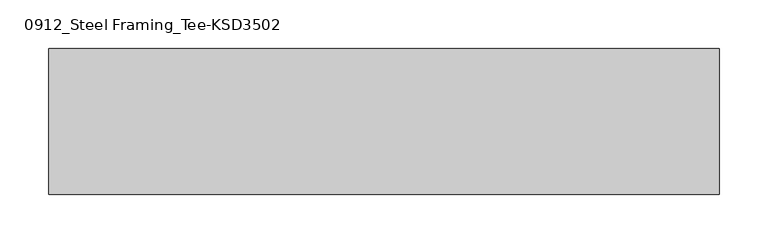
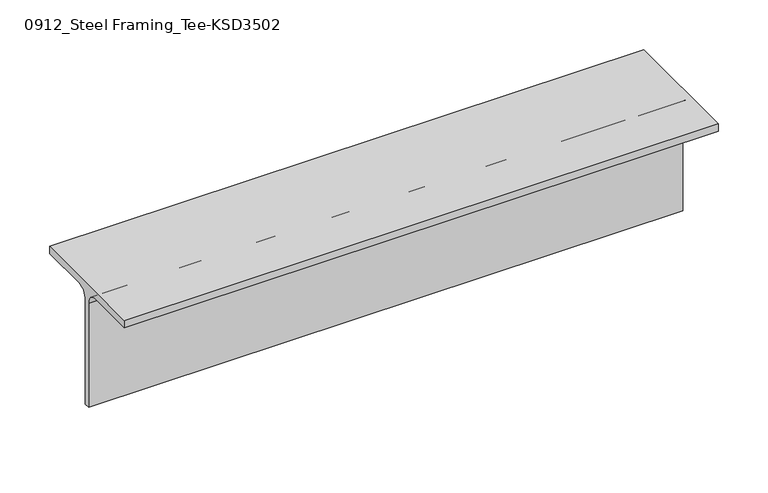
"""IFC4 building model written with IfcOpenShell, lengths in millimetres: member geometry, 0912_Steel Framing_Tee-KSD3502 : H_SB_ASB_CT-150x150x6.5x9."""

import ifcopenshell
import ifcopenshell.guid

model = None  # the IFC model being written
_history = None  # IfcOwnerHistory: only IFC2X3 demands one
_inside = {}  # id of a spatial element -> (the spatial element, [elements in it])
_under = {}  # id of a project, library or spatial element -> (it, [spatial elements below it])
_declared = {}  # id of a project -> (the project, [libraries it declares])
_typed = {}  # id of a type object -> (the type object, [elements of that type])
_made_of = {}  # id of a material, layer set ... -> (it, [elements and type objects made of it])


def new_model(schema):
    """Start an empty IFC model of exactly this schema.

    Asked for "IFC4X3", IfcOpenShell would pick the latest addendum, in which some entities
    have other attributes; the version numbers below select the first issue.
    IFC2X3 requires an IfcOwnerHistory on every rooted entity: one is made here for all.
    """
    global model, _history
    if schema == "IFC4X3":
        model = ifcopenshell.file(schema_version=(4, 3, 0, 0))
    else:
        model = ifcopenshell.file(schema=schema)
    _inside.clear()
    _under.clear()
    _declared.clear()
    _typed.clear()
    _made_of.clear()
    _history = None
    if model.schema == "IFC2X3":
        org = make("IfcOrganization", Name="unknown")
        user = make(
            "IfcPersonAndOrganization",
            ThePerson=make("IfcPerson", FamilyName="unknown"),
            TheOrganization=org,
        )
        app = make(
            "IfcApplication",
            ApplicationDeveloper=org,
            Version="unknown",
            ApplicationFullName="unknown",
            ApplicationIdentifier="unknown",
        )
        _history = make(
            "IfcOwnerHistory",
            OwningUser=user,
            OwningApplication=app,
            ChangeAction="ADDED",
            CreationDate=0,
        )
    return model


def make(cls, **values):
    """One entity of the class cls with the attributes given. An attribute that is None is left unset."""
    return model.create_entity(
        cls, **{name: value for name, value in values.items() if value is not None}
    )


def rooted(cls, **values):
    """An entity with a GlobalId (a new one), such as an element, a storey or a relation."""
    return make(cls, GlobalId=ifcopenshell.guid.new(), OwnerHistory=_history, **values)


def si_unit(unit_type, name, prefix=None):
    """IfcSIUnit, for example si_unit("LENGTHUNIT", "METRE", prefix="MILLI")."""
    return make("IfcSIUnit", UnitType=unit_type, Prefix=prefix, Name=name)


def assignment(units):
    """IfcUnitAssignment: the units of a project."""
    return None if units is None else make("IfcUnitAssignment", Units=units)


def point(xyz):
    """IfcCartesianPoint."""
    return None if xyz is None else make("IfcCartesianPoint", Coordinates=xyz)


def direction(xyz):
    """IfcDirection."""
    return None if xyz is None else make("IfcDirection", DirectionRatios=xyz)


def frame(location, z_axis=None, x_axis=None):
    """IfcAxis2Placement3D, a coordinate frame: its origin and axes. An axis left out is left unset."""
    return make(
        "IfcAxis2Placement3D",
        Location=point(location),
        Axis=direction(z_axis),
        RefDirection=direction(x_axis),
    )


def frame_2d(location, x_axis=None):
    """IfcAxis2Placement2D, a coordinate frame in the plane: its origin and x axis."""
    return make(
        "IfcAxis2Placement2D", Location=point(location), RefDirection=direction(x_axis)
    )


def origin():
    """The frame at (0, 0, 0) with its axes left unset."""
    return frame((0.0, 0.0, 0.0))


def place(relative_to, where):
    """IfcLocalPlacement: puts the frame where relative to a parent placement (None: the world)."""
    return make(
        "IfcLocalPlacement", PlacementRelTo=relative_to, RelativePlacement=where
    )


def context(
    kind, dimensions, precision=None, world=None, true_north=None, identifier=None
):
    """IfcGeometricRepresentationContext, for example the 3D "Model" context."""
    return make(
        "IfcGeometricRepresentationContext",
        ContextIdentifier=identifier,
        ContextType=kind,
        CoordinateSpaceDimension=dimensions,
        Precision=precision,
        WorldCoordinateSystem=world,
        TrueNorth=true_north,
    )


def project(units=None, contexts=None):
    """IfcProject with its units and contexts."""
    return rooted(
        "IfcProject",
        Name="project",
        RepresentationContexts=contexts,
        UnitsInContext=assignment(units),
    )


def spatial(cls, under=None, at=None, **own):
    """A site, building, storey or space (cls), placed at a placement, below another one or the project."""
    s = rooted(cls, ObjectPlacement=at, **own)
    if under is not None:
        _under.setdefault(under.id(), (under, []))[1].append(s)
    return s


def polyline(points):
    """IfcPolyline through the points."""
    return make("IfcPolyline", Points=[point(p) for p in points])


def circle_curve(where, radius):
    """IfcCircle in the frame where."""
    return make("IfcCircle", Position=where, Radius=radius)


def trimmed(basis, trim1, trim2, sense, master):
    """IfcTrimmedCurve: the piece of a basis curve between two trims."""
    return make(
        "IfcTrimmedCurve",
        BasisCurve=basis,
        Trim1=trim1,
        Trim2=trim2,
        SenseAgreement=sense,
        MasterRepresentation=master,
    )


def segment(curve, same_sense, transition):
    """IfcCompositeCurveSegment."""
    return make(
        "IfcCompositeCurveSegment",
        Transition=transition,
        SameSense=same_sense,
        ParentCurve=curve,
    )


def composite_curve(segments, self_intersect=None):
    """IfcCompositeCurve: segments joined end to end."""
    return make("IfcCompositeCurve", Segments=segments, SelfIntersect=self_intersect)


def outline(outer, holes=None, kind="AREA"):
    """IfcArbitraryClosedProfileDef: a profile drawn as a closed curve; with holes, ...WithVoids."""
    if holes is None:
        return make("IfcArbitraryClosedProfileDef", ProfileType=kind, OuterCurve=outer)
    return make(
        "IfcArbitraryProfileDefWithVoids",
        ProfileType=kind,
        OuterCurve=outer,
        InnerCurves=holes,
    )


def extrude(swept, where, along, depth):
    """IfcExtrudedAreaSolid: the profile swept, set in the frame where, extruded along a direction by depth."""
    return make(
        "IfcExtrudedAreaSolid",
        SweptArea=swept,
        Position=where,
        ExtrudedDirection=direction(along),
        Depth=depth,
    )


def shape(context_of_items, identifier, shape_type, items):
    """IfcShapeRepresentation: the items that make up one representation, for example the "Body"."""
    return make(
        "IfcShapeRepresentation",
        ContextOfItems=context_of_items,
        RepresentationIdentifier=identifier,
        RepresentationType=shape_type,
        Items=items,
    )


def source(mapping_origin, context_of_items, identifier, shape_type, items):
    """IfcRepresentationMap: a shape defined once, which mapped items show again and again."""
    return make(
        "IfcRepresentationMap",
        MappingOrigin=mapping_origin,
        MappedRepresentation=shape(context_of_items, identifier, shape_type, items),
    )


def transform(
    local_origin,
    x_axis=None,
    y_axis=None,
    z_axis=None,
    scale=None,
    scale2=None,
    scale3=None,
    uniform=True,
):
    """IfcCartesianTransformationOperator3D, or its non-uniform kind. x_axis, y_axis, z_axis: its Axis1, 2, 3."""
    if uniform:
        return make(
            "IfcCartesianTransformationOperator3D",
            Axis1=direction(x_axis),
            Axis2=direction(y_axis),
            LocalOrigin=point(local_origin),
            Scale=scale,
            Axis3=direction(z_axis),
        )
    return make(
        "IfcCartesianTransformationOperator3DnonUniform",
        Axis1=direction(x_axis),
        Axis2=direction(y_axis),
        LocalOrigin=point(local_origin),
        Scale=scale,
        Axis3=direction(z_axis),
        Scale2=scale2,
        Scale3=scale3,
    )


def mapped(mapping_source, mapping_target):
    """IfcMappedItem: shows the shape of a source again, moved by a transform."""
    return make(
        "IfcMappedItem", MappingSource=mapping_source, MappingTarget=mapping_target
    )


def made_of(thing, what):
    """Note that an element or type object is made of a material, layer set ...; save() writes the relation."""
    if what is not None:
        _made_of.setdefault(what.id(), (what, []))[1].append(thing)
    return thing


def element(
    cls,
    number,
    at=None,
    inside=None,
    cuts=None,
    type_object=None,
    material=None,
    context=None,
    identifier="Body",
    shape_type=None,
    held_by="IfcProductDefinitionShape",
    body=None,
    shapes=None,
    **own,
):
    """One element of the class cls, such as IfcWall. Its Tag is "e" and its number.

    at: its placement. inside: the storey or other place that contains it. cuts: it is an
    opening in that element (IfcRelVoidsElement). A single representation is given by context,
    identifier, shape_type and body (its items); several are given by shapes. held_by: the class
    of the entity that holds the representations. save() writes the other relations.
    """
    e = rooted(cls, Tag="e%d" % number, ObjectPlacement=at, **own)
    if body is not None:
        shapes = [shape(context, identifier, shape_type, body)]
    if shapes is not None:
        e.Representation = make(held_by, Representations=shapes)
    if inside is not None:
        _inside.setdefault(inside.id(), (inside, []))[1].append(e)
    if cuts is not None:
        rooted(
            "IfcRelVoidsElement", RelatingBuildingElement=cuts, RelatedOpeningElement=e
        )
    if type_object is not None:
        _typed.setdefault(type_object.id(), (type_object, []))[1].append(e)
    return made_of(e, material)


def aggregate(whole, parts):
    """IfcRelAggregates: a whole, such as a stair, and the parts it consists of."""
    return rooted("IfcRelAggregates", RelatingObject=whole, RelatedObjects=parts)


def save(model, path):
    """Write the relations noted so far, then the file.

    IfcRelAggregates (storeys below a building ...), IfcRelContainedInSpatialStructure (elements
    in a storey), IfcRelDefinesByType, IfcRelAssociatesMaterial and IfcRelDeclares: one each for
    every whole, place, type object, material and project.
    """
    for whole, parts in _under.values():
        aggregate(whole, parts)
    for where, things in _inside.values():
        rooted(
            "IfcRelContainedInSpatialStructure",
            RelatedElements=things,
            RelatingStructure=where,
        )
    for kind, things in _typed.values():
        rooted("IfcRelDefinesByType", RelatedObjects=things, RelatingType=kind)
    for what, things in _made_of.values():
        rooted("IfcRelAssociatesMaterial", RelatedObjects=things, RelatingMaterial=what)
    for by, libraries in _declared.values():
        rooted("IfcRelDeclares", RelatingContext=by, RelatedDefinitions=libraries)
    model.write(path)


def member_0912_steel_framing_tee_ksd3502_c00bb5e1(model_context):
    return source(origin(), model_context, "Body", "SweptSolid", [
        extrude(outline(composite_curve([segment(polyline([(-75.0, 75.0), (75.0, 75.0), (75.0, 66.0), (16.25, 66.0)]), True, "CONTINUOUS"), segment(trimmed(circle_curve(frame_2d((16.25, 53.0)), 13.0), [point((16.25, 66.0))], [point((3.25, 53.0))], True, "CARTESIAN"), True, "CONTINUOUS"), segment(polyline([(3.25, 53.0), (3.25, -75.0), (-3.25, -75.0), (-3.25, 53.0)]), True, "CONTINUOUS"), segment(trimmed(circle_curve(frame_2d((-16.25, 53.0)), 13.0), [point((-3.25, 53.0))], [point((-16.25, 66.0))], True, "CARTESIAN"), True, "CONTINUOUS"), segment(polyline([(-16.25, 66.0), (-75.0, 66.0), (-75.0, 75.0)]), True, "CONTINUOUS")], self_intersect=False)), frame((-335.8, 0.0, 0.0), z_axis=(1.0, 0.0, 0.0), x_axis=(0.0, 1.0, 0.0)), (0.0, 0.0, 1.0), 688.9),
    ])


if __name__ == "__main__":
    model = new_model("IFC4")
    model_context = context("Model", 3, world=origin())
    ifc_project = project(units=[si_unit("LENGTHUNIT", "METRE", prefix="MILLI")], contexts=[model_context])
    site = spatial("IfcSite", under=ifc_project)
    building = spatial("IfcBuilding", under=site)
    placement = place(None, origin())
    member_0912_steel_framing_tee_ksd3502_shape = member_0912_steel_framing_tee_ksd3502_c00bb5e1(model_context)
    element("IfcMember", 1, ObjectType="0912_Steel Framing_Tee-KSD3502 : H_SB_ASB_CT-150x150x6.5x9", at=placement, inside=building, context=model_context, shape_type="MappedRepresentation", body=[
        mapped(member_0912_steel_framing_tee_ksd3502_shape, transform((0.0, 0.0, 0.0), x_axis=(1.0, 0.0, 0.0), y_axis=(0.0, 1.0, 0.0), z_axis=(0.0, 0.0, 1.0))),
    ])
    save(model, "model.ifc")

# Revit data of these elements
# Type "0912_Steel Framing_Tee-KSD3502 : H_SB_ASB_CT-150x150x6.5x9"
#   H_WM Code_1 = "S01AA003-00001 | Main Steel Structure Fabrication Work | Shelter/Building | Light Steel - Standard (30KG/M>Weight) | Material: (   )"
#   H_WM Code_2 = "S03AA029-00001 | Main Steel Structure Erection Work | Shelter/Building | Light Steel (30KG/M>Weight) | Material: (   )"
#   H_WM Code_3 = "S01AA010-00001 | Main Steel Structure Fabrication Work | Shelter/Building | Steel Painting/Coating | for Non-Fireproofed Steel Surface, Surface Preparation, Primer, Second & Final Coat | Material: (   )"
#   H_Q'ty Cal Type Tag = "SB-Q2"
#   Width = 15.0 cm
#   Web Thickness = 0.65 cm
#   Web Fillet = 1.3 cm
#   Section Area = 23.39 cm²
#   Perimeter = 0.60 m²/m
#   Nominal Weight = 18.40 kgf/m
#   Height = 15.0 cm
#   Flange Thickness = 0.9 cm
#   Centroid Vertical = 7.5 cm
#   Centroid Horizontal = 7.5 cm
#   Length [instance default] = 1.5000 m
#   Structural Material [instance default] = Steel, 45-345
#   Warping Constant = (empty or 0)
#   Torsional Moment of Inertia = 0
#   Section Name Key = ""
#   Plastic Modulus weak axis = 0
#   Plastic Modulus strong axis = 0
#   Moment of Inertia weak axis = 0
#   Moment of Inertia strong axis = 0
#   Elastic Modulus weak axis = 0
#   Elastic Modulus strong axis = 0
#   Bolt Spacing = 0
#   Assembly Code = ""
# Element 1 (IfcMember, "0912_Steel Framing_Tee-KSD3502 : H_SB_ASB_CT-150x150x6.5x9")
#   Structural Material = none
# Materials
#   "Steel, 45-345": class "Metal", colour RGB 189 187 185, transparency 0, Description = "Steel 345 MPa", Cost = 0
